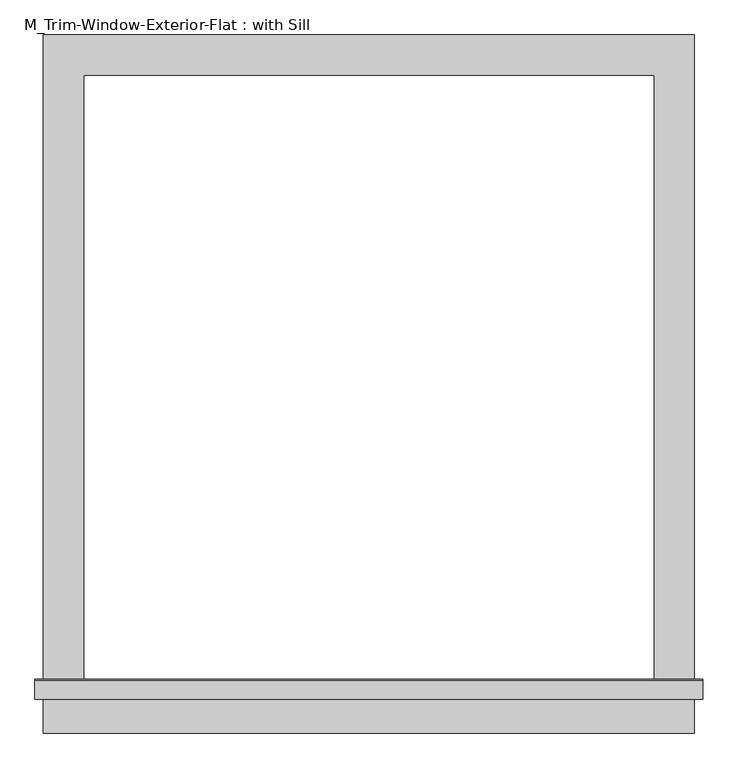
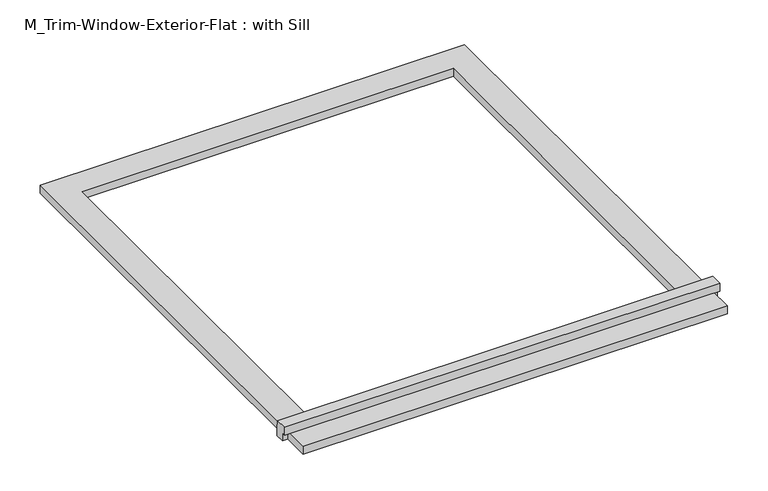
"""IFC4 building model written with IfcOpenShell, lengths in millimetres: proxy geometry, M_Trim-Window-Exterior-Flat : with Sill."""

import ifcopenshell
import ifcopenshell.guid

model = None  # the IFC model being written
_history = None  # IfcOwnerHistory: only IFC2X3 demands one
_inside = {}  # id of a spatial element -> (the spatial element, [elements in it])
_under = {}  # id of a project, library or spatial element -> (it, [spatial elements below it])
_declared = {}  # id of a project -> (the project, [libraries it declares])
_typed = {}  # id of a type object -> (the type object, [elements of that type])
_made_of = {}  # id of a material, layer set ... -> (it, [elements and type objects made of it])


def new_model(schema):
    """Start an empty IFC model of exactly this schema.

    Asked for "IFC4X3", IfcOpenShell would pick the latest addendum, in which some entities
    have other attributes; the version numbers below select the first issue.
    IFC2X3 requires an IfcOwnerHistory on every rooted entity: one is made here for all.
    """
    global model, _history
    if schema == "IFC4X3":
        model = ifcopenshell.file(schema_version=(4, 3, 0, 0))
    else:
        model = ifcopenshell.file(schema=schema)
    _inside.clear()
    _under.clear()
    _declared.clear()
    _typed.clear()
    _made_of.clear()
    _history = None
    if model.schema == "IFC2X3":
        org = make("IfcOrganization", Name="unknown")
        user = make(
            "IfcPersonAndOrganization",
            ThePerson=make("IfcPerson", FamilyName="unknown"),
            TheOrganization=org,
        )
        app = make(
            "IfcApplication",
            ApplicationDeveloper=org,
            Version="unknown",
            ApplicationFullName="unknown",
            ApplicationIdentifier="unknown",
        )
        _history = make(
            "IfcOwnerHistory",
            OwningUser=user,
            OwningApplication=app,
            ChangeAction="ADDED",
            CreationDate=0,
        )
    return model


def make(cls, **values):
    """One entity of the class cls with the attributes given. An attribute that is None is left unset."""
    return model.create_entity(
        cls, **{name: value for name, value in values.items() if value is not None}
    )


def rooted(cls, **values):
    """An entity with a GlobalId (a new one), such as an element, a storey or a relation."""
    return make(cls, GlobalId=ifcopenshell.guid.new(), OwnerHistory=_history, **values)


def si_unit(unit_type, name, prefix=None):
    """IfcSIUnit, for example si_unit("LENGTHUNIT", "METRE", prefix="MILLI")."""
    return make("IfcSIUnit", UnitType=unit_type, Prefix=prefix, Name=name)


def assignment(units):
    """IfcUnitAssignment: the units of a project."""
    return None if units is None else make("IfcUnitAssignment", Units=units)


def point(xyz):
    """IfcCartesianPoint."""
    return None if xyz is None else make("IfcCartesianPoint", Coordinates=xyz)


def direction(xyz):
    """IfcDirection."""
    return None if xyz is None else make("IfcDirection", DirectionRatios=xyz)


def frame(location, z_axis=None, x_axis=None):
    """IfcAxis2Placement3D, a coordinate frame: its origin and axes. An axis left out is left unset."""
    return make(
        "IfcAxis2Placement3D",
        Location=point(location),
        Axis=direction(z_axis),
        RefDirection=direction(x_axis),
    )


def origin():
    """The frame at (0, 0, 0) with its axes left unset."""
    return frame((0.0, 0.0, 0.0))


def origin_with_axes():
    """The frame at (0, 0, 0) with the z axis (0, 0, 1) and the x axis (1, 0, 0) written out."""
    return frame((0.0, 0.0, 0.0), z_axis=(0.0, 0.0, 1.0), x_axis=(1.0, 0.0, 0.0))


def place(relative_to, where):
    """IfcLocalPlacement: puts the frame where relative to a parent placement (None: the world)."""
    return make(
        "IfcLocalPlacement", PlacementRelTo=relative_to, RelativePlacement=where
    )


def context(
    kind, dimensions, precision=None, world=None, true_north=None, identifier=None
):
    """IfcGeometricRepresentationContext, for example the 3D "Model" context."""
    return make(
        "IfcGeometricRepresentationContext",
        ContextIdentifier=identifier,
        ContextType=kind,
        CoordinateSpaceDimension=dimensions,
        Precision=precision,
        WorldCoordinateSystem=world,
        TrueNorth=true_north,
    )


def project(units=None, contexts=None):
    """IfcProject with its units and contexts."""
    return rooted(
        "IfcProject",
        Name="project",
        RepresentationContexts=contexts,
        UnitsInContext=assignment(units),
    )


def spatial(cls, under=None, at=None, **own):
    """A site, building, storey or space (cls), placed at a placement, below another one or the project."""
    s = rooted(cls, ObjectPlacement=at, **own)
    if under is not None:
        _under.setdefault(under.id(), (under, []))[1].append(s)
    return s


def polyline(points):
    """IfcPolyline through the points."""
    return make("IfcPolyline", Points=[point(p) for p in points])


def outline(outer, holes=None, kind="AREA"):
    """IfcArbitraryClosedProfileDef: a profile drawn as a closed curve; with holes, ...WithVoids."""
    if holes is None:
        return make("IfcArbitraryClosedProfileDef", ProfileType=kind, OuterCurve=outer)
    return make(
        "IfcArbitraryProfileDefWithVoids",
        ProfileType=kind,
        OuterCurve=outer,
        InnerCurves=holes,
    )


def extrude(swept, where, along, depth):
    """IfcExtrudedAreaSolid: the profile swept, set in the frame where, extruded along a direction by depth."""
    return make(
        "IfcExtrudedAreaSolid",
        SweptArea=swept,
        Position=where,
        ExtrudedDirection=direction(along),
        Depth=depth,
    )


def shape(context_of_items, identifier, shape_type, items):
    """IfcShapeRepresentation: the items that make up one representation, for example the "Body"."""
    return make(
        "IfcShapeRepresentation",
        ContextOfItems=context_of_items,
        RepresentationIdentifier=identifier,
        RepresentationType=shape_type,
        Items=items,
    )


def source(mapping_origin, context_of_items, identifier, shape_type, items):
    """IfcRepresentationMap: a shape defined once, which mapped items show again and again."""
    return make(
        "IfcRepresentationMap",
        MappingOrigin=mapping_origin,
        MappedRepresentation=shape(context_of_items, identifier, shape_type, items),
    )


def transform(
    local_origin,
    x_axis=None,
    y_axis=None,
    z_axis=None,
    scale=None,
    scale2=None,
    scale3=None,
    uniform=True,
):
    """IfcCartesianTransformationOperator3D, or its non-uniform kind. x_axis, y_axis, z_axis: its Axis1, 2, 3."""
    if uniform:
        return make(
            "IfcCartesianTransformationOperator3D",
            Axis1=direction(x_axis),
            Axis2=direction(y_axis),
            LocalOrigin=point(local_origin),
            Scale=scale,
            Axis3=direction(z_axis),
        )
    return make(
        "IfcCartesianTransformationOperator3DnonUniform",
        Axis1=direction(x_axis),
        Axis2=direction(y_axis),
        LocalOrigin=point(local_origin),
        Scale=scale,
        Axis3=direction(z_axis),
        Scale2=scale2,
        Scale3=scale3,
    )


def mapped(mapping_source, mapping_target):
    """IfcMappedItem: shows the shape of a source again, moved by a transform."""
    return make(
        "IfcMappedItem", MappingSource=mapping_source, MappingTarget=mapping_target
    )


def made_of(thing, what):
    """Note that an element or type object is made of a material, layer set ...; save() writes the relation."""
    if what is not None:
        _made_of.setdefault(what.id(), (what, []))[1].append(thing)
    return thing


def element(
    cls,
    number,
    at=None,
    inside=None,
    cuts=None,
    type_object=None,
    material=None,
    context=None,
    identifier="Body",
    shape_type=None,
    held_by="IfcProductDefinitionShape",
    body=None,
    shapes=None,
    **own,
):
    """One element of the class cls, such as IfcWall. Its Tag is "e" and its number.

    at: its placement. inside: the storey or other place that contains it. cuts: it is an
    opening in that element (IfcRelVoidsElement). A single representation is given by context,
    identifier, shape_type and body (its items); several are given by shapes. held_by: the class
    of the entity that holds the representations. save() writes the other relations.
    """
    e = rooted(cls, Tag="e%d" % number, ObjectPlacement=at, **own)
    if body is not None:
        shapes = [shape(context, identifier, shape_type, body)]
    if shapes is not None:
        e.Representation = make(held_by, Representations=shapes)
    if inside is not None:
        _inside.setdefault(inside.id(), (inside, []))[1].append(e)
    if cuts is not None:
        rooted(
            "IfcRelVoidsElement", RelatingBuildingElement=cuts, RelatedOpeningElement=e
        )
    if type_object is not None:
        _typed.setdefault(type_object.id(), (type_object, []))[1].append(e)
    return made_of(e, material)


def aggregate(whole, parts):
    """IfcRelAggregates: a whole, such as a stair, and the parts it consists of."""
    return rooted("IfcRelAggregates", RelatingObject=whole, RelatedObjects=parts)


def save(model, path):
    """Write the relations noted so far, then the file.

    IfcRelAggregates (storeys below a building ...), IfcRelContainedInSpatialStructure (elements
    in a storey), IfcRelDefinesByType, IfcRelAssociatesMaterial and IfcRelDeclares: one each for
    every whole, place, type object, material and project.
    """
    for whole, parts in _under.values():
        aggregate(whole, parts)
    for where, things in _inside.values():
        rooted(
            "IfcRelContainedInSpatialStructure",
            RelatedElements=things,
            RelatingStructure=where,
        )
    for kind, things in _typed.values():
        rooted("IfcRelDefinesByType", RelatedObjects=things, RelatingType=kind)
    for what, things in _made_of.values():
        rooted("IfcRelAssociatesMaterial", RelatedObjects=things, RelatingMaterial=what)
    for by, libraries in _declared.values():
        rooted("IfcRelDeclares", RelatingContext=by, RelatedDefinitions=libraries)
    model.write(path)


def m_trim_window_exterior_flat_with_sill_90d3a428(model_context):
    return source(origin(), model_context, "Body", "SweptSolid", [
        extrude(outline(polyline([(485.0, -920.4323709), (485.0, -980.4323709), (-485.0, -980.4323709), (-485.0, -920.4323709), (485.0, -920.4323709)])), origin_with_axes(), (0.0, 0.0, 1.0), 19.05),
        extrude(outline(polyline([(-930.0, 38.1), (-902.4580645, 38.1), (-900.0, 19.05), (-900.0, 0.0), (-920.4323709, 0.0), (-920.4323709, 19.05), (-930.0, 19.05), (-930.0, 38.1)])), frame((-497.7, 0.0, 0.0), z_axis=(1.0, 0.0, 0.0), x_axis=(0.0, 1.0, 0.0)), (0.0, 0.0, 1.0), 995.4),
        extrude(outline(polyline([(-485.0, 60.0), (485.0, 60.0), (485.0, -900.0), (425.0, -900.0), (425.0, 0.0), (-425.0, 0.0), (-425.0, -900.0), (-485.0, -900.0), (-485.0, 60.0)])), origin_with_axes(), (0.0, 0.0, 1.0), 19.05),
    ])


if __name__ == "__main__":
    model = new_model("IFC4")
    model_context = context("Model", 3, world=origin())
    ifc_project = project(units=[si_unit("LENGTHUNIT", "METRE", prefix="MILLI")], contexts=[model_context])
    site = spatial("IfcSite", under=ifc_project)
    building = spatial("IfcBuilding", under=site)
    placement = place(None, origin())
    m_trim_window_exterior_flat_with_sill_shape = m_trim_window_exterior_flat_with_sill_90d3a428(model_context)
    element("IfcBuildingElementProxy", 1, Name="M_Trim-Window-Exterior-Flat : with Sill", ObjectType="M_Trim-Window-Exterior-Flat : with Sill", at=placement, inside=building, context=model_context, shape_type="MappedRepresentation", body=[
        mapped(m_trim_window_exterior_flat_with_sill_shape, transform((0.0, 0.0, 0.0), x_axis=(1.0, 0.0, 0.0), y_axis=(0.0, 1.0, 0.0), z_axis=(0.0, 0.0, 1.0))),
    ])
    save(model, "model.ifc")

# Revit data of these elements
# Type "M_Trim-Window-Exterior-Flat : with Sill"
#   Trim Width = 6 cm
#   Trim Thickness_Picture Frame = 3 cm
#   Trim Thickness_with Sill = 1.905 cm
#   Sill Thickness = 3 cm
#   Opening Width [instance default] = 60 cm
#   Opening Height [instance default] = 90 cm
#   Default Elevation = 120 cm
#   Sill = yes
#   Picture Frame = no
#   Trim Material [instance default] = none
# Element 1 (IfcBuildingElementProxy, "M_Trim-Window-Exterior-Flat : with Sill")
#   Opening Width = 85 cm
#   Trim Material = Clad - White
#   Materials on its faces: "Clad - White"
# Materials
#   "Clad - White": class "Wood", colour RGB 242 242 238, transparency 0, Cost = 0
